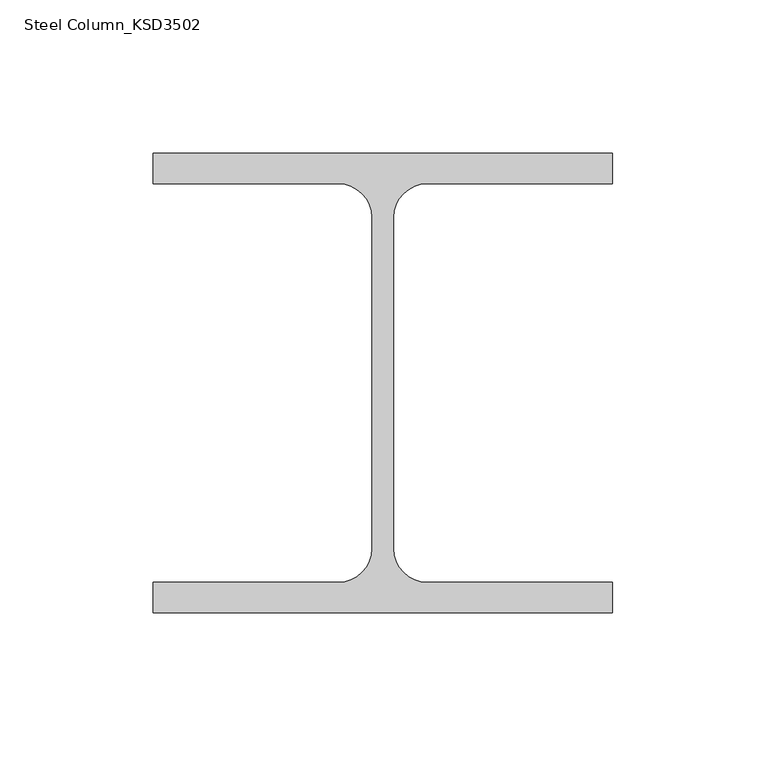
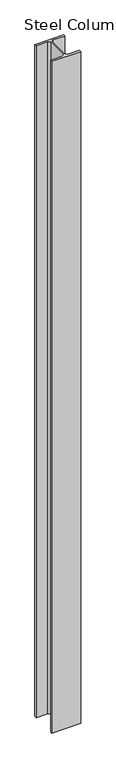
"""IFC4 building model written with IfcOpenShell, lengths in millimetres: column geometry, Steel Column_KSD3502 : H_SC_ASC_H-150×150x7x10."""

from ifc_helpers import new_model, si_unit, point, frame, frame_2d, origin, place, context, project, spatial, polyline, circle_curve, trimmed, segment, composite_curve, outline, extrude, source, transform, mapped, element, save


def steel_column_ksd3502_3e22cd7b(model_context):
    return source(origin(), model_context, "Body", "SweptSolid", [
        extrude(outline(composite_curve([segment(polyline([(75.0, 75.0), (75.0, 65.0), (14.5, 65.0)]), True, "CONTINUOUS"), segment(trimmed(circle_curve(frame_2d((14.5, 54.0)), 11.0), [point((14.5, 65.0))], [point((3.5, 54.0))], True, "CARTESIAN"), True, "CONTINUOUS"), segment(polyline([(3.5, 54.0), (3.5, -54.0)]), True, "CONTINUOUS"), segment(trimmed(circle_curve(frame_2d((14.5, -54.0)), 11.0), [point((3.5, -54.0))], [point((14.5, -65.0))], True, "CARTESIAN"), True, "CONTINUOUS"), segment(polyline([(14.5, -65.0), (75.0, -65.0), (75.0, -75.0), (-75.0, -75.0), (-75.0, -65.0), (-14.5, -65.0)]), True, "CONTINUOUS"), segment(trimmed(circle_curve(frame_2d((-14.5, -54.0)), 11.0), [point((-14.5, -65.0))], [point((-3.5, -54.0))], True, "CARTESIAN"), True, "CONTINUOUS"), segment(polyline([(-3.5, -54.0), (-3.5, 54.0)]), True, "CONTINUOUS"), segment(trimmed(circle_curve(frame_2d((-14.5, 54.0)), 11.0), [point((-3.5, 54.0))], [point((-14.5, 65.0))], True, "CARTESIAN"), True, "CONTINUOUS"), segment(polyline([(-14.5, 65.0), (-75.0, 65.0), (-75.0, 75.0), (75.0, 75.0)]), True, "CONTINUOUS")], self_intersect=False)), frame((0.0, 0.0, 599.9720055), z_axis=(0.0, 0.0, 1.0), x_axis=(1.0, 0.0, 0.0)), (0.0, 0.0, 1.0), 3678.0),
    ])


if __name__ == "__main__":
    model = new_model("IFC4")
    model_context = context("Model", 3, world=origin())
    ifc_project = project(units=[si_unit("LENGTHUNIT", "METRE", prefix="MILLI")], contexts=[model_context])
    site = spatial("IfcSite", under=ifc_project)
    building = spatial("IfcBuilding", under=site)
    placement = place(None, origin())
    steel_column_ksd3502_shape = steel_column_ksd3502_3e22cd7b(model_context)
    element("IfcColumn", 1, ObjectType="Steel Column_KSD3502 : H_SC_ASC_H-150×150x7x10", at=placement, inside=building, context=model_context, shape_type="MappedRepresentation", body=[
        mapped(steel_column_ksd3502_shape, transform((0.0, 0.0, 0.0), x_axis=(1.0, 0.0, 0.0), y_axis=(0.0, 1.0, 0.0), z_axis=(0.0, 0.0, 1.0))),
    ])
    save(model, "model.ifc")

# Revit data of these elements
# Type "Steel Column_KSD3502 : H_SC_ASC_H-150×150x7x10"
#   Width = 15.0 cm
#   Web Thickness = 0.7 cm
#   Web Fillet = 1.1 cm
#   Warping Constant = 27562.5 cm⁶
#   Torsional Moment of Inertia = 11.6007 cm⁴
#   Section Area = 40.14 cm²
#   Plastic Modulus weak axis = 115.0 cm³
#   Plastic Modulus strong axis = 246.0 cm³
#   Perimeter = 1.27 m²/m
#   Nominal Weight = 31.50 kgf/m
#   Moment of Inertia weak axis = 563.00 cm⁴
#   Moment of Inertia strong axis = 1640.00 cm⁴
#   Height = 15.0 cm
#   Flange Thickness = 1.0 cm
#   Elastic Modulus weak axis = 75.1 cm³
#   Elastic Modulus strong axis = 219.0 cm³
#   Centroid Vertical = 7.5 cm
#   Centroid Horizontal = 7.5 cm
#   Bolt Spacing = 13.97 cm
#   Structural Material [instance default] = Steel, 45-345
#   Section Name Key = ""
#   Assembly Code = ""
# Element 1 (IfcColumn, "Steel Column_KSD3502 : H_SC_ASC_H-150×150x7x10")
#   Structural Material = A03AD029-00005_Anchor Bolt (Installation only)_M24
#   Materials on its faces: "A03AD029-00005_Anchor Bolt (Installation only)_M24"
# Materials
#   "Steel, 45-345": class "Metal", colour RGB 189 187 185, transparency 0, Description = "Steel 345 MPa", Cost = 0
#   "A03AD029-00005_Anchor Bolt (Installation only)_M24": class "Unassigned", colour RGB 84 83 81, transparency 0, Cost = 0
